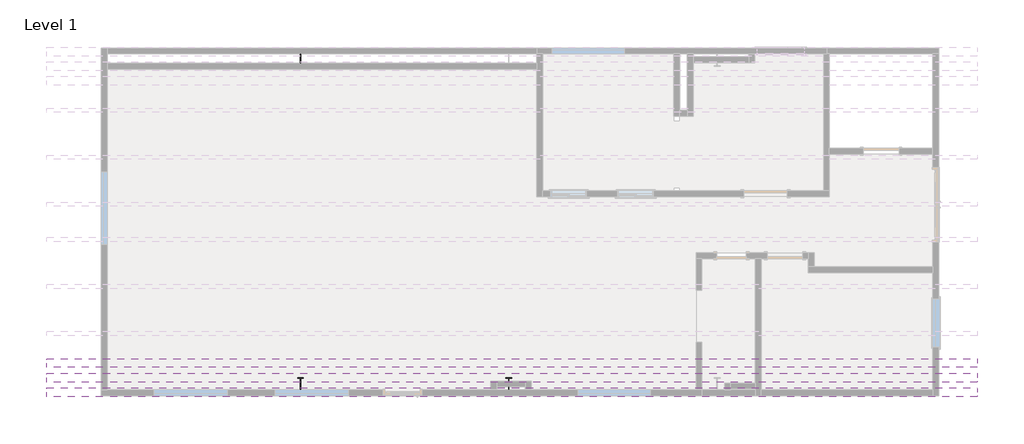
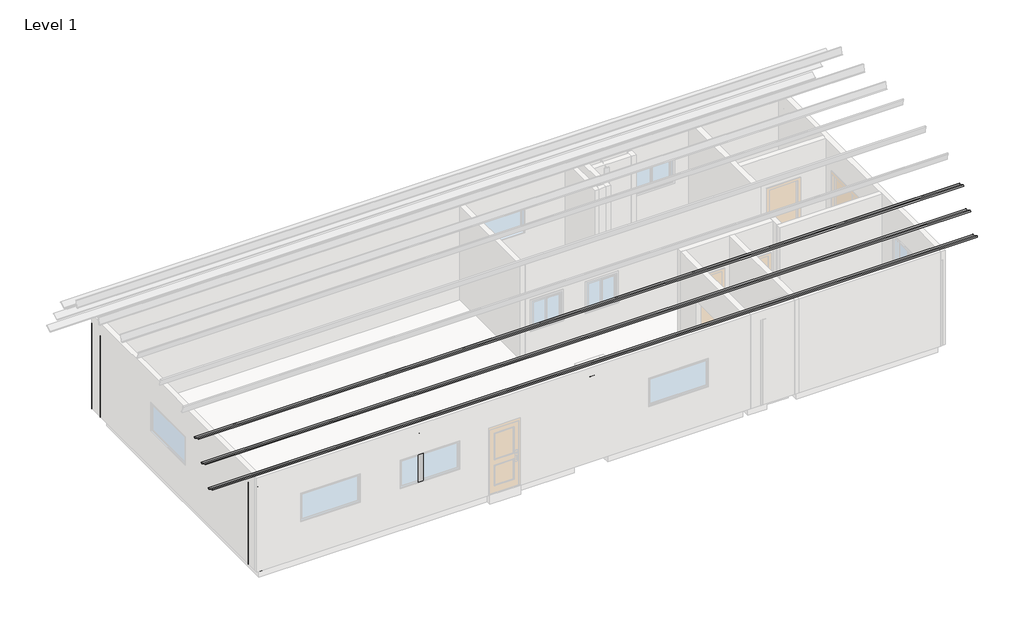
# One storey, part 2 of 3: 5 columns, 3 beams.
"""IFC4 building model written with IfcOpenShell, lengths in millimetres."""

import ifcopenshell
import ifcopenshell.guid

model = None  # the IFC model being written
_history = None  # IfcOwnerHistory: only IFC2X3 demands one
_inside = {}  # id of a spatial element -> (the spatial element, [elements in it])
_under = {}  # id of a project, library or spatial element -> (it, [spatial elements below it])
_declared = {}  # id of a project -> (the project, [libraries it declares])
_typed = {}  # id of a type object -> (the type object, [elements of that type])
_made_of = {}  # id of a material, layer set ... -> (it, [elements and type objects made of it])


def new_model(schema):
    """Start an empty IFC model of exactly this schema.

    Asked for "IFC4X3", IfcOpenShell would pick the latest addendum, in which some entities
    have other attributes; the version numbers below select the first issue.
    IFC2X3 requires an IfcOwnerHistory on every rooted entity: one is made here for all.
    """
    global model, _history
    if schema == "IFC4X3":
        model = ifcopenshell.file(schema_version=(4, 3, 0, 0))
    else:
        model = ifcopenshell.file(schema=schema)
    _inside.clear()
    _under.clear()
    _declared.clear()
    _typed.clear()
    _made_of.clear()
    _history = None
    if model.schema == "IFC2X3":
        org = make("IfcOrganization", Name="unknown")
        user = make(
            "IfcPersonAndOrganization",
            ThePerson=make("IfcPerson", FamilyName="unknown"),
            TheOrganization=org,
        )
        app = make(
            "IfcApplication",
            ApplicationDeveloper=org,
            Version="unknown",
            ApplicationFullName="unknown",
            ApplicationIdentifier="unknown",
        )
        _history = make(
            "IfcOwnerHistory",
            OwningUser=user,
            OwningApplication=app,
            ChangeAction="ADDED",
            CreationDate=0,
        )
    return model


def make(cls, **values):
    """One entity of the class cls with the attributes given. An attribute that is None is left unset."""
    return model.create_entity(
        cls, **{name: value for name, value in values.items() if value is not None}
    )


def rooted(cls, **values):
    """An entity with a GlobalId (a new one), such as an element, a storey or a relation."""
    return make(cls, GlobalId=ifcopenshell.guid.new(), OwnerHistory=_history, **values)


def si_unit(unit_type, name, prefix=None):
    """IfcSIUnit, for example si_unit("LENGTHUNIT", "METRE", prefix="MILLI")."""
    return make("IfcSIUnit", UnitType=unit_type, Prefix=prefix, Name=name)


def assignment(units):
    """IfcUnitAssignment: the units of a project."""
    return None if units is None else make("IfcUnitAssignment", Units=units)


def point(xyz):
    """IfcCartesianPoint."""
    return None if xyz is None else make("IfcCartesianPoint", Coordinates=xyz)


def direction(xyz):
    """IfcDirection."""
    return None if xyz is None else make("IfcDirection", DirectionRatios=xyz)


def frame(location, z_axis=None, x_axis=None):
    """IfcAxis2Placement3D, a coordinate frame: its origin and axes. An axis left out is left unset."""
    return make(
        "IfcAxis2Placement3D",
        Location=point(location),
        Axis=direction(z_axis),
        RefDirection=direction(x_axis),
    )


def origin():
    """The frame at (0, 0, 0) with its axes left unset."""
    return frame((0.0, 0.0, 0.0))


def place(relative_to, where):
    """IfcLocalPlacement: puts the frame where relative to a parent placement (None: the world)."""
    return make(
        "IfcLocalPlacement", PlacementRelTo=relative_to, RelativePlacement=where
    )


def context(
    kind, dimensions, precision=None, world=None, true_north=None, identifier=None
):
    """IfcGeometricRepresentationContext, for example the 3D "Model" context."""
    return make(
        "IfcGeometricRepresentationContext",
        ContextIdentifier=identifier,
        ContextType=kind,
        CoordinateSpaceDimension=dimensions,
        Precision=precision,
        WorldCoordinateSystem=world,
        TrueNorth=true_north,
    )


def project(units=None, contexts=None):
    """IfcProject with its units and contexts."""
    return rooted(
        "IfcProject",
        Name="project",
        RepresentationContexts=contexts,
        UnitsInContext=assignment(units),
    )


def spatial(cls, under=None, at=None, **own):
    """A site, building, storey or space (cls), placed at a placement, below another one or the project."""
    s = rooted(cls, ObjectPlacement=at, **own)
    if under is not None:
        _under.setdefault(under.id(), (under, []))[1].append(s)
    return s


def polyline(points):
    """IfcPolyline through the points."""
    return make("IfcPolyline", Points=[point(p) for p in points])


def circle_curve(where, radius):
    """IfcCircle in the frame where."""
    return make("IfcCircle", Position=where, Radius=radius)


def ellipse_curve(where, semi_axis1, semi_axis2):
    """IfcEllipse in the frame where."""
    return make(
        "IfcEllipse", Position=where, SemiAxis1=semi_axis1, SemiAxis2=semi_axis2
    )


def outline(outer, holes=None, kind="AREA"):
    """IfcArbitraryClosedProfileDef: a profile drawn as a closed curve; with holes, ...WithVoids."""
    if holes is None:
        return make("IfcArbitraryClosedProfileDef", ProfileType=kind, OuterCurve=outer)
    return make(
        "IfcArbitraryProfileDefWithVoids",
        ProfileType=kind,
        OuterCurve=outer,
        InnerCurves=holes,
    )


def extrude(swept, where, along, depth):
    """IfcExtrudedAreaSolid: the profile swept, set in the frame where, extruded along a direction by depth."""
    return make(
        "IfcExtrudedAreaSolid",
        SweptArea=swept,
        Position=where,
        ExtrudedDirection=direction(along),
        Depth=depth,
    )


def shape(context_of_items, identifier, shape_type, items):
    """IfcShapeRepresentation: the items that make up one representation, for example the "Body"."""
    return make(
        "IfcShapeRepresentation",
        ContextOfItems=context_of_items,
        RepresentationIdentifier=identifier,
        RepresentationType=shape_type,
        Items=items,
    )


def source(mapping_origin, context_of_items, identifier, shape_type, items):
    """IfcRepresentationMap: a shape defined once, which mapped items show again and again."""
    return make(
        "IfcRepresentationMap",
        MappingOrigin=mapping_origin,
        MappedRepresentation=shape(context_of_items, identifier, shape_type, items),
    )


def transform(
    local_origin,
    x_axis=None,
    y_axis=None,
    z_axis=None,
    scale=None,
    scale2=None,
    scale3=None,
    uniform=True,
):
    """IfcCartesianTransformationOperator3D, or its non-uniform kind. x_axis, y_axis, z_axis: its Axis1, 2, 3."""
    if uniform:
        return make(
            "IfcCartesianTransformationOperator3D",
            Axis1=direction(x_axis),
            Axis2=direction(y_axis),
            LocalOrigin=point(local_origin),
            Scale=scale,
            Axis3=direction(z_axis),
        )
    return make(
        "IfcCartesianTransformationOperator3DnonUniform",
        Axis1=direction(x_axis),
        Axis2=direction(y_axis),
        LocalOrigin=point(local_origin),
        Scale=scale,
        Axis3=direction(z_axis),
        Scale2=scale2,
        Scale3=scale3,
    )


def mapped(mapping_source, mapping_target):
    """IfcMappedItem: shows the shape of a source again, moved by a transform."""
    return make(
        "IfcMappedItem", MappingSource=mapping_source, MappingTarget=mapping_target
    )


def made_of(thing, what):
    """Note that an element or type object is made of a material, layer set ...; save() writes the relation."""
    if what is not None:
        _made_of.setdefault(what.id(), (what, []))[1].append(thing)
    return thing


def element(
    cls,
    number,
    at=None,
    inside=None,
    cuts=None,
    type_object=None,
    material=None,
    context=None,
    identifier="Body",
    shape_type=None,
    held_by="IfcProductDefinitionShape",
    body=None,
    shapes=None,
    **own,
):
    """One element of the class cls, such as IfcWall. Its Tag is "e" and its number.

    at: its placement. inside: the storey or other place that contains it. cuts: it is an
    opening in that element (IfcRelVoidsElement). A single representation is given by context,
    identifier, shape_type and body (its items); several are given by shapes. held_by: the class
    of the entity that holds the representations. save() writes the other relations.
    """
    e = rooted(cls, Tag="e%d" % number, ObjectPlacement=at, **own)
    if body is not None:
        shapes = [shape(context, identifier, shape_type, body)]
    if shapes is not None:
        e.Representation = make(held_by, Representations=shapes)
    if inside is not None:
        _inside.setdefault(inside.id(), (inside, []))[1].append(e)
    if cuts is not None:
        rooted(
            "IfcRelVoidsElement", RelatingBuildingElement=cuts, RelatedOpeningElement=e
        )
    if type_object is not None:
        _typed.setdefault(type_object.id(), (type_object, []))[1].append(e)
    return made_of(e, material)


def aggregate(whole, parts):
    """IfcRelAggregates: a whole, such as a stair, and the parts it consists of."""
    return rooted("IfcRelAggregates", RelatingObject=whole, RelatedObjects=parts)


def save(model, path):
    """Write the relations noted so far, then the file.

    IfcRelAggregates (storeys below a building ...), IfcRelContainedInSpatialStructure (elements
    in a storey), IfcRelDefinesByType, IfcRelAssociatesMaterial and IfcRelDeclares: one each for
    every whole, place, type object, material and project.
    """
    for whole, parts in _under.values():
        aggregate(whole, parts)
    for where, things in _inside.values():
        rooted(
            "IfcRelContainedInSpatialStructure",
            RelatedElements=things,
            RelatingStructure=where,
        )
    for kind, things in _typed.values():
        rooted("IfcRelDefinesByType", RelatedObjects=things, RelatingType=kind)
    for what, things in _made_of.values():
        rooted("IfcRelAssociatesMaterial", RelatedObjects=things, RelatingMaterial=what)
    for by, libraries in _declared.values():
        rooted("IfcRelDeclares", RelatingContext=by, RelatedDefinitions=libraries)
    model.write(path)


def plane_surface(at):
    """IfcPlane: the flat surface through the origin of the frame at, square to its z axis."""
    return make("IfcPlane", Position=at)


def revolved_surface(curve, axis_point, axis_direction):
    """IfcSurfaceOfRevolution: the curve turned about the line through axis_point along axis_direction."""
    return make(
        "IfcSurfaceOfRevolution",
        SweptCurve=make("IfcArbitraryOpenProfileDef", ProfileType="CURVE", Curve=curve),
        AxisPosition=make("IfcAxis1Placement", Location=point(axis_point), Axis=direction(axis_direction)),
    )


def advanced_brep(points, edges, surfaces, faces):
    """IfcAdvancedBrep: a solid bounded by faces that lie on surfaces and meet in shared edges.

    An edge is (start, end): straight between two places in points (the first is 0);
    or (start, end, curve); or (start, end, curve, False) where it runs against its curve.
    A face is (place in surfaces, loops), or (place, loops, False) where it looks against
    its surface's normal. A loop lists edges by number (the first is 1), with a minus sign
    where the edge is run from its end to its start. The first loop is the outer one.
    """
    corners = [point(p) for p in points]
    vertices = [make("IfcVertexPoint", VertexGeometry=c) for c in corners]
    made = []
    for start, end, *more in edges:
        made.append(
            make(
                "IfcEdgeCurve",
                EdgeStart=vertices[start],
                EdgeEnd=vertices[end],
                EdgeGeometry=more[0] if more else make("IfcPolyline", Points=[corners[start], corners[end]]),
                SameSense=more[1] if len(more) > 1 else True,
            )
        )
    hull = []
    for where, loops, *sense in faces:
        bounds = []
        for j, loop in enumerate(loops):
            ring = [make("IfcOrientedEdge", EdgeElement=made[abs(k) - 1], Orientation=k > 0) for k in loop]
            bounds.append(
                make(
                    "IfcFaceOuterBound" if j == 0 else "IfcFaceBound",
                    Bound=make("IfcEdgeLoop", EdgeList=ring),
                    Orientation=True,
                )
            )
        hull.append(make("IfcAdvancedFace", Bounds=bounds, FaceSurface=surfaces[where], SameSense=sense[0] if sense else True))
    return make("IfcAdvancedBrep", Outer=make("IfcClosedShell", CfsFaces=hull))


def z_shapes_z_3x8_0ff4bf34(model_context):
    return source(origin(), model_context, "Body", "SweptSolid", [
        extrude(outline(polyline([(-57.2805719, 101.596825), (-57.2805719, 111.248825), (-19.1805719, 111.248825), (-19.1805719, -101.603175), (18.9194281, -101.603175), (18.9194281, -107.953175), (-27.1991352, -107.953175), (-27.1991352, 101.596825), (-57.2805719, 101.596825)])), frame((-11963.4, 0.0, 0.0), z_axis=(1.0, 0.0, 0.0), x_axis=(0.0, 1.0, 0.0)), (0.0, 0.0, 1.0), 23926.8),
    ])


model = new_model("IFC4")

# Units and contexts
model_context = context("Model", 3, world=origin())
ifc_project = project(units=[si_unit("LENGTHUNIT", "METRE", prefix="MILLI")], contexts=[model_context])

# Site, building, storey
site = spatial("IfcSite", under=ifc_project)
building = spatial("IfcBuilding", under=site)
storey = spatial("IfcBuildingStorey", under=building, Name="Level 1", Elevation=0.0)

# Beams
placement = place(None, origin())
z_shapes_z_3x8_shape = z_shapes_z_3x8_0ff4bf34(model_context)
element("IfcBeam", 1, ObjectType="Z Shapes : Z 3X8", at=placement, inside=storey, context=model_context, shape_type="MappedRepresentation", body=[
    mapped(z_shapes_z_3x8_shape, transform((18060.1870052, 3496.8149514, 4436.794501), x_axis=(1.0, 0.0, 0.0), y_axis=(0.0, 0.5198738321222879, 0.8542430559708913), z_axis=(0.0, -0.8542430559708913, 0.5198738321222879))),
])
element("IfcBeam", 2, ObjectType="Z Shapes : Z 3X8", at=placement, inside=storey, context=model_context, shape_type="MappedRepresentation", body=[
    mapped(z_shapes_z_3x8_shape, transform((18060.1870052, 3122.2539613, 3821.3256987), x_axis=(1.0, 0.0, 0.0), y_axis=(0.0, 0.5198738321222879, 0.8542430559708913), z_axis=(0.0, -0.8542430559708913, 0.5198738321222879))),
])
element("IfcBeam", 3, ObjectType="Z Shapes : Z 3X8", at=placement, inside=storey, context=model_context, shape_type="MappedRepresentation", body=[
    mapped(z_shapes_z_3x8_shape, transform((18060.1870052, 2747.6929713, 3205.8568965), x_axis=(1.0, 0.0, 0.0), y_axis=(0.0, 0.5198738321222879, 0.8542430559708913), z_axis=(0.0, -0.8542430559708913, 0.5198738321222879))),
])

# Columns
element("IfcColumn", 4, ObjectType="W-Wide Flange-Column : W6X18.5", at=placement, inside=storey, context=model_context, shape_type="AdvancedBrep", body=[
    advanced_brep(
    [(17901.4370052, 2642.8615366, 0.0), (17901.4370052, 2653.1485366, 0.0), (17962.3970052, 2653.1485366, 0.0), (17974.3350052, 2665.0865366, 0.0), (17974.3350052, 3090.5365366, 0.0), (17962.3970052, 3102.4745366, 0.0), (17901.4370052, 3102.4745366, 0.0), (17901.4370052, 3112.7615366, 0.0), (18053.8370052, 3112.7615366, 0.0), (18053.8370052, 3102.4745366, 0.0), (17992.8770052, 3102.4745366, 0.0), (17980.9390052, 3090.5365366, 0.0), (17980.9390052, 2665.0865366, 0.0), (17992.8770052, 2653.1485366, 0.0), (18053.8370052, 2653.1485366, 0.0), (18053.8370052, 2642.8615366, 0.0), (17901.4370052, 2642.8615366, 2825.947988), (17901.4370052, 2653.1485366, 2823.0639572), (17962.3970052, 2653.1485366, 2823.0639572), (17974.3350052, 2665.0865366, 2819.7170571), (17974.3350052, 3090.5365366, 2700.4392375), (17962.3970052, 3102.4745366, 2697.0923375), (17901.4370052, 3102.4745366, 2697.0923375), (17901.4370052, 3112.7615366, 2694.2083066), (18053.8370052, 3112.7615366, 2694.2083066), (18053.8370052, 3102.4745366, 2697.0923375), (17992.8770052, 3102.4745366, 2697.0923375), (17980.9390052, 3090.5365366, 2700.4392375), (17980.9390052, 2665.0865366, 2819.7170571), (17992.8770052, 2653.1485366, 2823.0639572), (18053.8370052, 2653.1485366, 2823.0639572), (18053.8370052, 2642.8615366, 2825.947988)],
    [
        (0, 1),
        (1, 2),
        (2, 3, circle_curve(frame((17962.3970052, 2665.0865366, 0.0), z_axis=(0.0, 0.0, 1.0), x_axis=(-1.0, 0.0, 0.0)), 11.938)),
        (3, 4),
        (4, 5, circle_curve(frame((17962.3970052, 3090.5365366, 0.0), z_axis=(0.0, 0.0, 1.0), x_axis=(-1.0, 0.0, 0.0)), 11.938)),
        (5, 6),
        (6, 7),
        (7, 8),
        (8, 9),
        (9, 10),
        (10, 11, circle_curve(frame((17992.8770052, 3090.5365366, 0.0), z_axis=(0.0, 0.0, 1.0), x_axis=(-1.0, 0.0, 0.0)), 11.938)),
        (11, 12),
        (12, 13, circle_curve(frame((17992.8770052, 2665.0865366, 0.0), z_axis=(0.0, 0.0, 1.0), x_axis=(-1.0, 0.0, 0.0)), 11.938)),
        (13, 14),
        (14, 15),
        (15, 0),
        (0, 16),
        (16, 17),
        (17, 1),
        (17, 18),
        (18, 2),
        (18, 19, ellipse_curve(frame((17962.3970052, 2665.0865366, 2819.7170571), z_axis=(0.0, 0.2699485280248201, 0.962874754169634), x_axis=(0.0, 0.962874754169634, -0.26994852802481967)), 12.3982895, 11.938)),
        (19, 3),
        (19, 20),
        (20, 4),
        (20, 21, ellipse_curve(frame((17962.3970052, 3090.5365366, 2700.4392375), z_axis=(0.0, 0.2699485280248201, 0.962874754169634), x_axis=(0.0, 0.962874754169634, -0.26994852802481967)), 12.3982895, 11.938)),
        (21, 5),
        (21, 22),
        (22, 6),
        (22, 23),
        (23, 7),
        (23, 24),
        (24, 8),
        (24, 25),
        (25, 9),
        (25, 26),
        (26, 10),
        (26, 27, ellipse_curve(frame((17992.8770052, 3090.5365366, 2700.4392375), z_axis=(0.0, 0.2699485280248201, 0.962874754169634), x_axis=(0.0, 0.962874754169634, -0.26994852802481967)), 12.3982895, 11.938)),
        (27, 11),
        (27, 28),
        (28, 12),
        (28, 29, ellipse_curve(frame((17992.8770052, 2665.0865366, 2819.7170571), z_axis=(0.0, 0.2699485280248201, 0.962874754169634), x_axis=(0.0, 0.962874754169634, -0.26994852802481967)), 12.3982895, 11.938)),
        (29, 13),
        (29, 30),
        (30, 14),
        (30, 31),
        (31, 15),
        (31, 16),
    ],
    [
        plane_surface(frame((18053.8370052, 2642.8615366, 0.0), z_axis=(0.0, 0.0, -1.0), x_axis=(-1.0, 0.0, 0.0))),
        plane_surface(frame((17901.4370052, 2653.1485366, 2832.1), z_axis=(-1.0, 0.0, 0.0), x_axis=(0.0, 0.0, -1.0))),
        plane_surface(frame((17962.3970052, 2653.1485366, 2832.1), z_axis=(0.0, 1.0, 0.0), x_axis=(0.0, 0.0, -1.0))),
        revolved_surface(polyline([(17950.459005200002, 2665.0865366, 0.0), (17950.459005200002, 2665.0865366, 2823.0639572)]), (17962.3970052, 2665.0865366, 0.0), (0.0, 0.0, -1.0)),
        plane_surface(frame((17974.3350052, 3090.5365366, 2832.1), z_axis=(-1.0, 0.0, 0.0), x_axis=(0.0, 0.0, -1.0))),
        revolved_surface(polyline([(17950.459005200002, 3090.5365366, 0.0), (17950.459005200002, 3090.5365366, 2703.786137500551)]), (17962.3970052, 3090.5365366, 0.0), (0.0, 0.0, -1.0)),
        plane_surface(frame((17901.4370052, 3102.4745366, 2832.1), z_axis=(0.0, -1.0, 0.0), x_axis=(0.0, 0.0, -1.0))),
        plane_surface(frame((17901.4370052, 3112.7615366, 2832.1), z_axis=(-1.0, 0.0, 0.0), x_axis=(0.0, 0.0, -1.0))),
        plane_surface(frame((18053.8370052, 3112.7615366, 2832.1), z_axis=(0.0, 1.0, 0.0), x_axis=(0.0, 0.0, -1.0))),
        plane_surface(frame((18053.8370052, 3102.4745366, 2832.1), z_axis=(1.0, 0.0, 0.0), x_axis=(0.0, 0.0, -1.0))),
        plane_surface(frame((17992.8770052, 3102.4745366, 2832.1), z_axis=(0.0, -1.0, 0.0), x_axis=(0.0, 0.0, -1.0))),
        revolved_surface(polyline([(17980.9390052, 3090.5365366, 0.0), (17980.9390052, 3090.5365366, 2703.786137500551)]), (17992.8770052, 3090.5365366, 0.0), (0.0, 0.0, -1.0)),
        plane_surface(frame((17980.9390052, 2665.0865366, 2832.1), z_axis=(1.0, 0.0, 0.0), x_axis=(0.0, 0.0, -1.0))),
        revolved_surface(polyline([(17980.9390052, 2665.0865366, 0.0), (17980.9390052, 2665.0865366, 2823.0639572)]), (17992.8770052, 2665.0865366, 0.0), (0.0, 0.0, -1.0)),
        plane_surface(frame((18053.8370052, 2653.1485366, 2832.1), z_axis=(0.0, 1.0, 0.0), x_axis=(0.0, 0.0, -1.0))),
        plane_surface(frame((18053.8370052, 2642.8615366, 2832.1), z_axis=(1.0, 0.0, 0.0), x_axis=(0.0, 0.0, -1.0))),
        plane_surface(frame((17901.4370052, 2642.8615366, 2832.1), z_axis=(0.0, -1.0, 0.0), x_axis=(0.0, 0.0, -1.0))),
        plane_surface(frame((20809.7370052, 2504.5013556, 2864.7382118), z_axis=(0.0, 0.2699485280248201, 0.962874754169634), x_axis=(-1.0, 0.0, 0.0))),
    ],
    [
        (0, [[1, 2, 3, 4, 5, 6, 7, 8, 9, 10, 11, 12, 13, 14, 15, 16]]),
        (1, [[-1, 17, 18, 19]]),
        (2, [[-2, -19, 20, 21]]),
        (3, [[-3, -21, 22, 23]]),
        (4, [[-4, -23, 24, 25]]),
        (5, [[-5, -25, 26, 27]]),
        (6, [[-6, -27, 28, 29]]),
        (7, [[-7, -29, 30, 31]]),
        (8, [[-8, -31, 32, 33]]),
        (9, [[-9, -33, 34, 35]]),
        (10, [[-10, -35, 36, 37]]),
        (11, [[-11, -37, 38, 39]]),
        (12, [[-12, -39, 40, 41]]),
        (13, [[-13, -41, 42, 43]]),
        (14, [[-14, -43, 44, 45]]),
        (15, [[-15, -45, 46, 47]]),
        (16, [[-16, -47, 48, -17]]),
        (17, [[-18, -48, -46, -44, -42, -40, -38, -36, -34, -32, -30, -28, -26, -24, -22, -20]]),
    ],
),
])
element("IfcColumn", 5, ObjectType="W-Wide Flange-Column : W6X18.5", at=placement, inside=storey, context=model_context, shape_type="AdvancedBrep", body=[
    advanced_brep(
    [(12700.7870052, 11583.6615366, 0.0), (12700.7870052, 11573.3745366, 0.0), (12639.8270052, 11573.3745366, 0.0), (12627.8890052, 11561.4365366, 0.0), (12627.8890052, 11135.9865366, 0.0), (12639.8270052, 11124.0485366, 0.0), (12700.7870052, 11124.0485366, 0.0), (12700.7870052, 11113.7615366, 0.0), (12548.3870052, 11113.7615366, 0.0), (12548.3870052, 11124.0485366, 0.0), (12609.3470052, 11124.0485366, 0.0), (12621.2850052, 11135.9865366, 0.0), (12621.2850052, 11561.4365366, 0.0), (12609.3470052, 11573.3745366, 0.0), (12548.3870052, 11573.3745366, 0.0), (12548.3870052, 11583.6615366, 0.0), (12700.7870052, 11583.6615366, 2825.947988), (12700.7870052, 11573.3745366, 2823.0639572), (12639.8270052, 11573.3745366, 2823.0639572), (12627.8890052, 11561.4365366, 2819.7170571), (12627.8890052, 11135.9865366, 2700.4392375), (12639.8270052, 11124.0485366, 2697.0923375), (12700.7870052, 11124.0485366, 2697.0923375), (12700.7870052, 11113.7615366, 2694.2083066), (12548.3870052, 11113.7615366, 2694.2083066), (12548.3870052, 11124.0485366, 2697.0923375), (12609.3470052, 11124.0485366, 2697.0923375), (12621.2850052, 11135.9865366, 2700.4392375), (12621.2850052, 11561.4365366, 2819.7170571), (12609.3470052, 11573.3745366, 2823.0639572), (12548.3870052, 11573.3745366, 2823.0639572), (12548.3870052, 11583.6615366, 2825.947988)],
    [
        (0, 1),
        (1, 2),
        (2, 3, circle_curve(frame((12639.8270052, 11561.4365366, 0.0), z_axis=(0.0, 0.0, 1.0), x_axis=(1.0, 0.0, 0.0)), 11.938)),
        (3, 4),
        (4, 5, circle_curve(frame((12639.8270052, 11135.9865366, 0.0), z_axis=(0.0, 0.0, 1.0), x_axis=(1.0, 0.0, 0.0)), 11.938)),
        (5, 6),
        (6, 7),
        (7, 8),
        (8, 9),
        (9, 10),
        (10, 11, circle_curve(frame((12609.3470052, 11135.9865366, 0.0), z_axis=(0.0, 0.0, 1.0), x_axis=(1.0, 0.0, 0.0)), 11.938)),
        (11, 12),
        (12, 13, circle_curve(frame((12609.3470052, 11561.4365366, 0.0), z_axis=(0.0, 0.0, 1.0), x_axis=(1.0, 0.0, 0.0)), 11.938)),
        (13, 14),
        (14, 15),
        (15, 0),
        (0, 16),
        (16, 17),
        (17, 1),
        (17, 18),
        (18, 2),
        (18, 19, ellipse_curve(frame((12639.8270052, 11561.4365366, 2819.7170571), z_axis=(0.0, -0.26994852802481994, 0.962874754169634), x_axis=(0.0, -0.9628747541696339, -0.26994852802481983)), 12.3982895, 11.938)),
        (19, 3),
        (19, 20),
        (20, 4),
        (20, 21, ellipse_curve(frame((12639.8270052, 11135.9865366, 2700.4392375), z_axis=(0.0, -0.26994852802481994, 0.962874754169634), x_axis=(0.0, -0.9628747541696339, -0.26994852802481983)), 12.3982895, 11.938)),
        (21, 5),
        (21, 22),
        (22, 6),
        (22, 23),
        (23, 7),
        (23, 24),
        (24, 8),
        (24, 25),
        (25, 9),
        (25, 26),
        (26, 10),
        (26, 27, ellipse_curve(frame((12609.3470052, 11135.9865366, 2700.4392375), z_axis=(0.0, -0.26994852802481994, 0.962874754169634), x_axis=(0.0, -0.9628747541696339, -0.26994852802481983)), 12.3982895, 11.938)),
        (27, 11),
        (27, 28),
        (28, 12),
        (28, 29, ellipse_curve(frame((12609.3470052, 11561.4365366, 2819.7170571), z_axis=(0.0, -0.26994852802481994, 0.962874754169634), x_axis=(0.0, -0.9628747541696339, -0.26994852802481983)), 12.3982895, 11.938)),
        (29, 13),
        (29, 30),
        (30, 14),
        (30, 31),
        (31, 15),
        (31, 16),
    ],
    [
        plane_surface(frame((12548.3870052, 11583.6615366, 0.0), z_axis=(0.0, 0.0, -1.0), x_axis=(1.0, 0.0, 0.0))),
        plane_surface(frame((12700.7870052, 11573.3745366, 2832.1), z_axis=(1.0, 0.0, 0.0), x_axis=(0.0, 0.0, -1.0))),
        plane_surface(frame((12639.8270052, 11573.3745366, 2832.1), z_axis=(0.0, -1.0, 0.0), x_axis=(0.0, 0.0, -1.0))),
        revolved_surface(polyline([(12651.7650052, 11561.4365366, 0.0), (12651.7650052, 11561.4365366, 2823.0639572)]), (12639.8270052, 11561.4365366, 0.0), (0.0, 0.0, -1.0)),
        plane_surface(frame((12627.8890052, 11135.9865366, 2832.1), z_axis=(1.0, 0.0, 0.0), x_axis=(0.0, 0.0, -1.0))),
        revolved_surface(polyline([(12651.7650052, 11135.9865366, 0.0), (12651.7650052, 11135.9865366, 2703.786137500551)]), (12639.8270052, 11135.9865366, 0.0), (0.0, 0.0, -1.0)),
        plane_surface(frame((12700.7870052, 11124.0485366, 2832.1), z_axis=(0.0, 1.0, 0.0), x_axis=(0.0, 0.0, -1.0))),
        plane_surface(frame((12700.7870052, 11113.7615366, 2832.1), z_axis=(1.0, 0.0, 0.0), x_axis=(0.0, 0.0, -1.0))),
        plane_surface(frame((12548.3870052, 11113.7615366, 2832.1), z_axis=(0.0, -1.0, 0.0), x_axis=(0.0, 0.0, -1.0))),
        plane_surface(frame((12548.3870052, 11124.0485366, 2832.1), z_axis=(-1.0, 0.0, 0.0), x_axis=(0.0, 0.0, -1.0))),
        plane_surface(frame((12609.3470052, 11124.0485366, 2832.1), z_axis=(0.0, 1.0, 0.0), x_axis=(0.0, 0.0, -1.0))),
        revolved_surface(polyline([(12621.2850052, 11135.9865366, 0.0), (12621.2850052, 11135.9865366, 2703.786137500551)]), (12609.3470052, 11135.9865366, 0.0), (0.0, 0.0, -1.0)),
        plane_surface(frame((12621.2850052, 11561.4365366, 2832.1), z_axis=(-1.0, 0.0, 0.0), x_axis=(0.0, 0.0, -1.0))),
        revolved_surface(polyline([(12621.2850052, 11561.4365366, 0.0), (12621.2850052, 11561.4365366, 2823.0639572)]), (12609.3470052, 11561.4365366, 0.0), (0.0, 0.0, -1.0)),
        plane_surface(frame((12548.3870052, 11573.3745366, 2832.1), z_axis=(0.0, -1.0, 0.0), x_axis=(0.0, 0.0, -1.0))),
        plane_surface(frame((12548.3870052, 11583.6615366, 2832.1), z_axis=(-1.0, 0.0, 0.0), x_axis=(0.0, 0.0, -1.0))),
        plane_surface(frame((12700.7870052, 11583.6615366, 2832.1), z_axis=(0.0, 1.0, 0.0), x_axis=(0.0, 0.0, -1.0))),
        plane_surface(frame((9792.4870052, 11722.0217176, 2864.7382118), z_axis=(0.0, -0.26994852802481994, 0.962874754169634), x_axis=(1.0, 0.0, 0.0))),
    ],
    [
        (0, [[1, 2, 3, 4, 5, 6, 7, 8, 9, 10, 11, 12, 13, 14, 15, 16]]),
        (1, [[-1, 17, 18, 19]]),
        (2, [[-2, -19, 20, 21]]),
        (3, [[-3, -21, 22, 23]]),
        (4, [[-4, -23, 24, 25]]),
        (5, [[-5, -25, 26, 27]]),
        (6, [[-6, -27, 28, 29]]),
        (7, [[-7, -29, 30, 31]]),
        (8, [[-8, -31, 32, 33]]),
        (9, [[-9, -33, 34, 35]]),
        (10, [[-10, -35, 36, 37]]),
        (11, [[-11, -37, 38, 39]]),
        (12, [[-12, -39, 40, 41]]),
        (13, [[-13, -41, 42, 43]]),
        (14, [[-14, -43, 44, 45]]),
        (15, [[-15, -45, 46, 47]]),
        (16, [[-16, -47, 48, -17]]),
        (17, [[-18, -48, -46, -44, -42, -40, -38, -36, -34, -32, -30, -28, -26, -24, -22, -20]]),
    ],
),
])
element("IfcColumn", 6, ObjectType="W-Wide Flange-Column : W6X18.5", at=placement, inside=storey, context=model_context, shape_type="AdvancedBrep", body=[
    advanced_brep(
    [(12548.3870052, 2642.8615366, 0.0), (12548.3870052, 2653.1485366, 0.0), (12609.3470052, 2653.1485366, 0.0), (12621.2850052, 2665.0865366, 0.0), (12621.2850052, 3090.5365366, 0.0), (12609.3470052, 3102.4745366, 0.0), (12548.3870052, 3102.4745366, 0.0), (12548.3870052, 3112.7615366, 0.0), (12700.7870052, 3112.7615366, 0.0), (12700.7870052, 3102.4745366, 0.0), (12639.8270052, 3102.4745366, 0.0), (12627.8890052, 3090.5365366, 0.0), (12627.8890052, 2665.0865366, 0.0), (12639.8270052, 2653.1485366, 0.0), (12700.7870052, 2653.1485366, 0.0), (12700.7870052, 2642.8615366, 0.0), (12548.3870052, 2642.8615366, 2825.947988), (12548.3870052, 2653.1485366, 2823.0639572), (12609.3470052, 2653.1485366, 2823.0639572), (12621.2850052, 2665.0865366, 2819.7170571), (12621.2850052, 3090.5365366, 2700.4392375), (12609.3470052, 3102.4745366, 2697.0923375), (12548.3870052, 3102.4745366, 2697.0923375), (12548.3870052, 3112.7615366, 2694.2083066), (12700.7870052, 3112.7615366, 2694.2083066), (12700.7870052, 3102.4745366, 2697.0923375), (12639.8270052, 3102.4745366, 2697.0923375), (12627.8890052, 3090.5365366, 2700.4392375), (12627.8890052, 2665.0865366, 2819.7170571), (12639.8270052, 2653.1485366, 2823.0639572), (12700.7870052, 2653.1485366, 2823.0639572), (12700.7870052, 2642.8615366, 2825.947988)],
    [
        (0, 1),
        (1, 2),
        (2, 3, circle_curve(frame((12609.3470052, 2665.0865366, 0.0), z_axis=(0.0, 0.0, 1.0), x_axis=(-1.0, 0.0, 0.0)), 11.938)),
        (3, 4),
        (4, 5, circle_curve(frame((12609.3470052, 3090.5365366, 0.0), z_axis=(0.0, 0.0, 1.0), x_axis=(-1.0, 0.0, 0.0)), 11.938)),
        (5, 6),
        (6, 7),
        (7, 8),
        (8, 9),
        (9, 10),
        (10, 11, circle_curve(frame((12639.8270052, 3090.5365366, 0.0), z_axis=(0.0, 0.0, 1.0), x_axis=(-1.0, 0.0, 0.0)), 11.938)),
        (11, 12),
        (12, 13, circle_curve(frame((12639.8270052, 2665.0865366, 0.0), z_axis=(0.0, 0.0, 1.0), x_axis=(-1.0, 0.0, 0.0)), 11.938)),
        (13, 14),
        (14, 15),
        (15, 0),
        (0, 16),
        (16, 17),
        (17, 1),
        (17, 18),
        (18, 2),
        (18, 19, ellipse_curve(frame((12609.3470052, 2665.0865366, 2819.7170571), z_axis=(0.0, 0.2699485280248201, 0.962874754169634), x_axis=(0.0, 0.962874754169634, -0.26994852802481967)), 12.3982895, 11.938)),
        (19, 3),
        (19, 20),
        (20, 4),
        (20, 21, ellipse_curve(frame((12609.3470052, 3090.5365366, 2700.4392375), z_axis=(0.0, 0.2699485280248201, 0.962874754169634), x_axis=(0.0, 0.962874754169634, -0.26994852802481967)), 12.3982895, 11.938)),
        (21, 5),
        (21, 22),
        (22, 6),
        (22, 23),
        (23, 7),
        (23, 24),
        (24, 8),
        (24, 25),
        (25, 9),
        (25, 26),
        (26, 10),
        (26, 27, ellipse_curve(frame((12639.8270052, 3090.5365366, 2700.4392375), z_axis=(0.0, 0.2699485280248201, 0.962874754169634), x_axis=(0.0, 0.962874754169634, -0.26994852802481967)), 12.3982895, 11.938)),
        (27, 11),
        (27, 28),
        (28, 12),
        (28, 29, ellipse_curve(frame((12639.8270052, 2665.0865366, 2819.7170571), z_axis=(0.0, 0.2699485280248201, 0.962874754169634), x_axis=(0.0, 0.962874754169634, -0.26994852802481967)), 12.3982895, 11.938)),
        (29, 13),
        (29, 30),
        (30, 14),
        (30, 31),
        (31, 15),
        (31, 16),
    ],
    [
        plane_surface(frame((12700.7870052, 2642.8615366, 0.0), z_axis=(0.0, 0.0, -1.0), x_axis=(-1.0, 0.0, 0.0))),
        plane_surface(frame((12548.3870052, 2653.1485366, 2832.1), z_axis=(-1.0, 0.0, 0.0), x_axis=(0.0, 0.0, -1.0))),
        plane_surface(frame((12609.3470052, 2653.1485366, 2832.1), z_axis=(0.0, 1.0, 0.0), x_axis=(0.0, 0.0, -1.0))),
        revolved_surface(polyline([(12597.4090052, 2665.0865366, 0.0), (12597.4090052, 2665.0865366, 2823.0639572)]), (12609.3470052, 2665.0865366, 0.0), (0.0, 0.0, -1.0)),
        plane_surface(frame((12621.2850052, 3090.5365366, 2832.1), z_axis=(-1.0, 0.0, 0.0), x_axis=(0.0, 0.0, -1.0))),
        revolved_surface(polyline([(12597.4090052, 3090.5365366, 0.0), (12597.4090052, 3090.5365366, 2703.786137500551)]), (12609.3470052, 3090.5365366, 0.0), (0.0, 0.0, -1.0)),
        plane_surface(frame((12548.3870052, 3102.4745366, 2832.1), z_axis=(0.0, -1.0, 0.0), x_axis=(0.0, 0.0, -1.0))),
        plane_surface(frame((12548.3870052, 3112.7615366, 2832.1), z_axis=(-1.0, 0.0, 0.0), x_axis=(0.0, 0.0, -1.0))),
        plane_surface(frame((12700.7870052, 3112.7615366, 2832.1), z_axis=(0.0, 1.0, 0.0), x_axis=(0.0, 0.0, -1.0))),
        plane_surface(frame((12700.7870052, 3102.4745366, 2832.1), z_axis=(1.0, 0.0, 0.0), x_axis=(0.0, 0.0, -1.0))),
        plane_surface(frame((12639.8270052, 3102.4745366, 2832.1), z_axis=(0.0, -1.0, 0.0), x_axis=(0.0, 0.0, -1.0))),
        revolved_surface(polyline([(12627.8890052, 3090.5365366, 0.0), (12627.8890052, 3090.5365366, 2703.786137500551)]), (12639.8270052, 3090.5365366, 0.0), (0.0, 0.0, -1.0)),
        plane_surface(frame((12627.8890052, 2665.0865366, 2832.1), z_axis=(1.0, 0.0, 0.0), x_axis=(0.0, 0.0, -1.0))),
        revolved_surface(polyline([(12627.8890052, 2665.0865366, 0.0), (12627.8890052, 2665.0865366, 2823.0639572)]), (12639.8270052, 2665.0865366, 0.0), (0.0, 0.0, -1.0)),
        plane_surface(frame((12700.7870052, 2653.1485366, 2832.1), z_axis=(0.0, 1.0, 0.0), x_axis=(0.0, 0.0, -1.0))),
        plane_surface(frame((12700.7870052, 2642.8615366, 2832.1), z_axis=(1.0, 0.0, 0.0), x_axis=(0.0, 0.0, -1.0))),
        plane_surface(frame((12548.3870052, 2642.8615366, 2832.1), z_axis=(0.0, -1.0, 0.0), x_axis=(0.0, 0.0, -1.0))),
        plane_surface(frame((15456.6870052, 2504.5013556, 2864.7382118), z_axis=(0.0, 0.2699485280248201, 0.962874754169634), x_axis=(-1.0, 0.0, 0.0))),
    ],
    [
        (0, [[1, 2, 3, 4, 5, 6, 7, 8, 9, 10, 11, 12, 13, 14, 15, 16]]),
        (1, [[-1, 17, 18, 19]]),
        (2, [[-2, -19, 20, 21]]),
        (3, [[-3, -21, 22, 23]]),
        (4, [[-4, -23, 24, 25]]),
        (5, [[-5, -25, 26, 27]]),
        (6, [[-6, -27, 28, 29]]),
        (7, [[-7, -29, 30, 31]]),
        (8, [[-8, -31, 32, 33]]),
        (9, [[-9, -33, 34, 35]]),
        (10, [[-10, -35, 36, 37]]),
        (11, [[-11, -37, 38, 39]]),
        (12, [[-12, -39, 40, 41]]),
        (13, [[-13, -41, 42, 43]]),
        (14, [[-14, -43, 44, 45]]),
        (15, [[-15, -45, 46, 47]]),
        (16, [[-16, -47, 48, -17]]),
        (17, [[-18, -48, -46, -44, -42, -40, -38, -36, -34, -32, -30, -28, -26, -24, -22, -20]]),
    ],
),
])
element("IfcColumn", 7, ObjectType="W-Wide Flange-Column : W6X18.5", at=placement, inside=storey, context=model_context, shape_type="AdvancedBrep", body=[
    advanced_brep(
    [(7652.5405771, 11583.6615366, 0.0), (7652.5405771, 11573.3745366, 0.0), (7591.5805771, 11573.3745366, 0.0), (7579.6425771, 11561.4365366, 0.0), (7579.6425771, 11135.9865366, 0.0), (7591.5805771, 11124.0485366, 0.0), (7652.5405771, 11124.0485366, 0.0), (7652.5405771, 11113.7615366, 0.0), (7500.1405771, 11113.7615366, 0.0), (7500.1405771, 11124.0485366, 0.0), (7561.1005771, 11124.0485366, 0.0), (7573.0385771, 11135.9865366, 0.0), (7573.0385771, 11561.4365366, 0.0), (7561.1005771, 11573.3745366, 0.0), (7500.1405771, 11573.3745366, 0.0), (7500.1405771, 11583.6615366, 0.0), (7652.5405771, 11583.6615366, 2825.947988), (7652.5405771, 11573.3745366, 2823.0639572), (7591.5805771, 11573.3745366, 2823.0639572), (7579.6425771, 11561.4365366, 2819.7170571), (7579.6425771, 11135.9865366, 2700.4392375), (7591.5805771, 11124.0485366, 2697.0923375), (7652.5405771, 11124.0485366, 2697.0923375), (7652.5405771, 11113.7615366, 2694.2083066), (7500.1405771, 11113.7615366, 2694.2083066), (7500.1405771, 11124.0485366, 2697.0923375), (7561.1005771, 11124.0485366, 2697.0923375), (7573.0385771, 11135.9865366, 2700.4392375), (7573.0385771, 11561.4365366, 2819.7170571), (7561.1005771, 11573.3745366, 2823.0639572), (7500.1405771, 11573.3745366, 2823.0639572), (7500.1405771, 11583.6615366, 2825.947988)],
    [
        (0, 1),
        (1, 2),
        (2, 3, circle_curve(frame((7591.5805771, 11561.4365366, 0.0), z_axis=(0.0, 0.0, 1.0), x_axis=(1.0, 0.0, 0.0)), 11.938)),
        (3, 4),
        (4, 5, circle_curve(frame((7591.5805771, 11135.9865366, 0.0), z_axis=(0.0, 0.0, 1.0), x_axis=(1.0, 0.0, 0.0)), 11.938)),
        (5, 6),
        (6, 7),
        (7, 8),
        (8, 9),
        (9, 10),
        (10, 11, circle_curve(frame((7561.1005771, 11135.9865366, 0.0), z_axis=(0.0, 0.0, 1.0), x_axis=(1.0, 0.0, 0.0)), 11.938)),
        (11, 12),
        (12, 13, circle_curve(frame((7561.1005771, 11561.4365366, 0.0), z_axis=(0.0, 0.0, 1.0), x_axis=(1.0, 0.0, 0.0)), 11.938)),
        (13, 14),
        (14, 15),
        (15, 0),
        (0, 16),
        (16, 17),
        (17, 1),
        (17, 18),
        (18, 2),
        (18, 19, ellipse_curve(frame((7591.5805771, 11561.4365366, 2819.7170571), z_axis=(0.0, -0.26994852802481994, 0.962874754169634), x_axis=(0.0, -0.9628747541696339, -0.26994852802481983)), 12.3982895, 11.938)),
        (19, 3),
        (19, 20),
        (20, 4),
        (20, 21, ellipse_curve(frame((7591.5805771, 11135.9865366, 2700.4392375), z_axis=(0.0, -0.26994852802481994, 0.962874754169634), x_axis=(0.0, -0.9628747541696339, -0.26994852802481983)), 12.3982895, 11.938)),
        (21, 5),
        (21, 22),
        (22, 6),
        (22, 23),
        (23, 7),
        (23, 24),
        (24, 8),
        (24, 25),
        (25, 9),
        (25, 26),
        (26, 10),
        (26, 27, ellipse_curve(frame((7561.1005771, 11135.9865366, 2700.4392375), z_axis=(0.0, -0.26994852802481994, 0.962874754169634), x_axis=(0.0, -0.9628747541696339, -0.26994852802481983)), 12.3982895, 11.938)),
        (27, 11),
        (27, 28),
        (28, 12),
        (28, 29, ellipse_curve(frame((7561.1005771, 11561.4365366, 2819.7170571), z_axis=(0.0, -0.26994852802481994, 0.962874754169634), x_axis=(0.0, -0.9628747541696339, -0.26994852802481983)), 12.3982895, 11.938)),
        (29, 13),
        (29, 30),
        (30, 14),
        (30, 31),
        (31, 15),
        (31, 16),
    ],
    [
        plane_surface(frame((7500.1405771, 11583.6615366, 0.0), z_axis=(0.0, 0.0, -1.0), x_axis=(1.0, 0.0, 0.0))),
        plane_surface(frame((7652.5405771, 11573.3745366, 2832.1), z_axis=(1.0, 0.0, 0.0), x_axis=(0.0, 0.0, -1.0))),
        plane_surface(frame((7591.5805771, 11573.3745366, 2832.1), z_axis=(0.0, -1.0, 0.0), x_axis=(0.0, 0.0, -1.0))),
        revolved_surface(polyline([(7603.5185771, 11561.4365366, 0.0), (7603.5185771, 11561.4365366, 2823.0639572)]), (7591.5805771, 11561.4365366, 0.0), (0.0, 0.0, -1.0)),
        plane_surface(frame((7579.6425771, 11135.9865366, 2832.1), z_axis=(1.0, 0.0, 0.0), x_axis=(0.0, 0.0, -1.0))),
        revolved_surface(polyline([(7603.5185771, 11135.9865366, 0.0), (7603.5185771, 11135.9865366, 2703.786137500551)]), (7591.5805771, 11135.9865366, 0.0), (0.0, 0.0, -1.0)),
        plane_surface(frame((7652.5405771, 11124.0485366, 2832.1), z_axis=(0.0, 1.0, 0.0), x_axis=(0.0, 0.0, -1.0))),
        plane_surface(frame((7652.5405771, 11113.7615366, 2832.1), z_axis=(1.0, 0.0, 0.0), x_axis=(0.0, 0.0, -1.0))),
        plane_surface(frame((7500.1405771, 11113.7615366, 2832.1), z_axis=(0.0, -1.0, 0.0), x_axis=(0.0, 0.0, -1.0))),
        plane_surface(frame((7500.1405771, 11124.0485366, 2832.1), z_axis=(-1.0, 0.0, 0.0), x_axis=(0.0, 0.0, -1.0))),
        plane_surface(frame((7561.1005771, 11124.0485366, 2832.1), z_axis=(0.0, 1.0, 0.0), x_axis=(0.0, 0.0, -1.0))),
        revolved_surface(polyline([(7573.0385771, 11135.9865366, 0.0), (7573.0385771, 11135.9865366, 2703.786137500551)]), (7561.1005771, 11135.9865366, 0.0), (0.0, 0.0, -1.0)),
        plane_surface(frame((7573.0385771, 11561.4365366, 2832.1), z_axis=(-1.0, 0.0, 0.0), x_axis=(0.0, 0.0, -1.0))),
        revolved_surface(polyline([(7573.0385771, 11561.4365366, 0.0), (7573.0385771, 11561.4365366, 2823.0639572)]), (7561.1005771, 11561.4365366, 0.0), (0.0, 0.0, -1.0)),
        plane_surface(frame((7500.1405771, 11573.3745366, 2832.1), z_axis=(0.0, -1.0, 0.0), x_axis=(0.0, 0.0, -1.0))),
        plane_surface(frame((7500.1405771, 11583.6615366, 2832.1), z_axis=(-1.0, 0.0, 0.0), x_axis=(0.0, 0.0, -1.0))),
        plane_surface(frame((7652.5405771, 11583.6615366, 2832.1), z_axis=(0.0, 1.0, 0.0), x_axis=(0.0, 0.0, -1.0))),
        plane_surface(frame((4744.2405771, 11722.0217176, 2864.7382118), z_axis=(0.0, -0.26994852802481994, 0.962874754169634), x_axis=(1.0, 0.0, 0.0))),
    ],
    [
        (0, [[1, 2, 3, 4, 5, 6, 7, 8, 9, 10, 11, 12, 13, 14, 15, 16]]),
        (1, [[-1, 17, 18, 19]]),
        (2, [[-2, -19, 20, 21]]),
        (3, [[-3, -21, 22, 23]]),
        (4, [[-4, -23, 24, 25]]),
        (5, [[-5, -25, 26, 27]]),
        (6, [[-6, -27, 28, 29]]),
        (7, [[-7, -29, 30, 31]]),
        (8, [[-8, -31, 32, 33]]),
        (9, [[-9, -33, 34, 35]]),
        (10, [[-10, -35, 36, 37]]),
        (11, [[-11, -37, 38, 39]]),
        (12, [[-12, -39, 40, 41]]),
        (13, [[-13, -41, 42, 43]]),
        (14, [[-14, -43, 44, 45]]),
        (15, [[-15, -45, 46, 47]]),
        (16, [[-16, -47, 48, -17]]),
        (17, [[-18, -48, -46, -44, -42, -40, -38, -36, -34, -32, -30, -28, -26, -24, -22, -20]]),
    ],
),
])
element("IfcColumn", 8, ObjectType="W-Wide Flange-Column : W6X18.5", at=placement, inside=storey, context=model_context, shape_type="AdvancedBrep", body=[
    advanced_brep(
    [(7500.1405771, 2642.8615366, 0.0), (7500.1405771, 2653.1485366, 0.0), (7561.1005771, 2653.1485366, 0.0), (7573.0385771, 2665.0865366, 0.0), (7573.0385771, 3090.5365366, 0.0), (7561.1005771, 3102.4745366, 0.0), (7500.1405771, 3102.4745366, 0.0), (7500.1405771, 3112.7615366, 0.0), (7652.5405771, 3112.7615366, 0.0), (7652.5405771, 3102.4745366, 0.0), (7591.5805771, 3102.4745366, 0.0), (7579.6425771, 3090.5365366, 0.0), (7579.6425771, 2665.0865366, 0.0), (7591.5805771, 2653.1485366, 0.0), (7652.5405771, 2653.1485366, 0.0), (7652.5405771, 2642.8615366, 0.0), (7500.1405771, 2642.8615366, 2825.947988), (7500.1405771, 2653.1485366, 2823.0639572), (7561.1005771, 2653.1485366, 2823.0639572), (7573.0385771, 2665.0865366, 2819.7170571), (7573.0385771, 3090.5365366, 2700.4392375), (7561.1005771, 3102.4745366, 2697.0923375), (7500.1405771, 3102.4745366, 2697.0923375), (7500.1405771, 3112.7615366, 2694.2083066), (7652.5405771, 3112.7615366, 2694.2083066), (7652.5405771, 3102.4745366, 2697.0923375), (7591.5805771, 3102.4745366, 2697.0923375), (7579.6425771, 3090.5365366, 2700.4392375), (7579.6425771, 2665.0865366, 2819.7170571), (7591.5805771, 2653.1485366, 2823.0639572), (7652.5405771, 2653.1485366, 2823.0639572), (7652.5405771, 2642.8615366, 2825.947988)],
    [
        (0, 1),
        (1, 2),
        (2, 3, circle_curve(frame((7561.1005771, 2665.0865366, 0.0), z_axis=(0.0, 0.0, 1.0), x_axis=(-1.0, 0.0, 0.0)), 11.938)),
        (3, 4),
        (4, 5, circle_curve(frame((7561.1005771, 3090.5365366, 0.0), z_axis=(0.0, 0.0, 1.0), x_axis=(-1.0, 0.0, 0.0)), 11.938)),
        (5, 6),
        (6, 7),
        (7, 8),
        (8, 9),
        (9, 10),
        (10, 11, circle_curve(frame((7591.5805771, 3090.5365366, 0.0), z_axis=(0.0, 0.0, 1.0), x_axis=(-1.0, 0.0, 0.0)), 11.938)),
        (11, 12),
        (12, 13, circle_curve(frame((7591.5805771, 2665.0865366, 0.0), z_axis=(0.0, 0.0, 1.0), x_axis=(-1.0, 0.0, 0.0)), 11.938)),
        (13, 14),
        (14, 15),
        (15, 0),
        (0, 16),
        (16, 17),
        (17, 1),
        (17, 18),
        (18, 2),
        (18, 19, ellipse_curve(frame((7561.1005771, 2665.0865366, 2819.7170571), z_axis=(0.0, 0.2699485280248201, 0.962874754169634), x_axis=(0.0, 0.962874754169634, -0.26994852802481967)), 12.3982895, 11.938)),
        (19, 3),
        (19, 20),
        (20, 4),
        (20, 21, ellipse_curve(frame((7561.1005771, 3090.5365366, 2700.4392375), z_axis=(0.0, 0.2699485280248201, 0.962874754169634), x_axis=(0.0, 0.962874754169634, -0.26994852802481967)), 12.3982895, 11.938)),
        (21, 5),
        (21, 22),
        (22, 6),
        (22, 23),
        (23, 7),
        (23, 24),
        (24, 8),
        (24, 25),
        (25, 9),
        (25, 26),
        (26, 10),
        (26, 27, ellipse_curve(frame((7591.5805771, 3090.5365366, 2700.4392375), z_axis=(0.0, 0.2699485280248201, 0.962874754169634), x_axis=(0.0, 0.962874754169634, -0.26994852802481967)), 12.3982895, 11.938)),
        (27, 11),
        (27, 28),
        (28, 12),
        (28, 29, ellipse_curve(frame((7591.5805771, 2665.0865366, 2819.7170571), z_axis=(0.0, 0.2699485280248201, 0.962874754169634), x_axis=(0.0, 0.962874754169634, -0.26994852802481967)), 12.3982895, 11.938)),
        (29, 13),
        (29, 30),
        (30, 14),
        (30, 31),
        (31, 15),
        (31, 16),
    ],
    [
        plane_surface(frame((7652.5405771, 2642.8615366, 0.0), z_axis=(0.0, 0.0, -1.0), x_axis=(-1.0, 0.0, 0.0))),
        plane_surface(frame((7500.1405771, 2653.1485366, 2832.1), z_axis=(-1.0, 0.0, 0.0), x_axis=(0.0, 0.0, -1.0))),
        plane_surface(frame((7561.1005771, 2653.1485366, 2832.1), z_axis=(0.0, 1.0, 0.0), x_axis=(0.0, 0.0, -1.0))),
        revolved_surface(polyline([(7549.1625771, 2665.0865366, 0.0), (7549.1625771, 2665.0865366, 2823.0639572)]), (7561.1005771, 2665.0865366, 0.0), (0.0, 0.0, -1.0)),
        plane_surface(frame((7573.0385771, 3090.5365366, 2832.1), z_axis=(-1.0, 0.0, 0.0), x_axis=(0.0, 0.0, -1.0))),
        revolved_surface(polyline([(7549.1625771, 3090.5365366, 0.0), (7549.1625771, 3090.5365366, 2703.786137500551)]), (7561.1005771, 3090.5365366, 0.0), (0.0, 0.0, -1.0)),
        plane_surface(frame((7500.1405771, 3102.4745366, 2832.1), z_axis=(0.0, -1.0, 0.0), x_axis=(0.0, 0.0, -1.0))),
        plane_surface(frame((7500.1405771, 3112.7615366, 2832.1), z_axis=(-1.0, 0.0, 0.0), x_axis=(0.0, 0.0, -1.0))),
        plane_surface(frame((7652.5405771, 3112.7615366, 2832.1), z_axis=(0.0, 1.0, 0.0), x_axis=(0.0, 0.0, -1.0))),
        plane_surface(frame((7652.5405771, 3102.4745366, 2832.1), z_axis=(1.0, 0.0, 0.0), x_axis=(0.0, 0.0, -1.0))),
        plane_surface(frame((7591.5805771, 3102.4745366, 2832.1), z_axis=(0.0, -1.0, 0.0), x_axis=(0.0, 0.0, -1.0))),
        revolved_surface(polyline([(7579.6425770999995, 3090.5365366, 0.0), (7579.6425770999995, 3090.5365366, 2703.786137500551)]), (7591.5805771, 3090.5365366, 0.0), (0.0, 0.0, -1.0)),
        plane_surface(frame((7579.6425771, 2665.0865366, 2832.1), z_axis=(1.0, 0.0, 0.0), x_axis=(0.0, 0.0, -1.0))),
        revolved_surface(polyline([(7579.6425770999995, 2665.0865366, 0.0), (7579.6425770999995, 2665.0865366, 2823.0639572)]), (7591.5805771, 2665.0865366, 0.0), (0.0, 0.0, -1.0)),
        plane_surface(frame((7652.5405771, 2653.1485366, 2832.1), z_axis=(0.0, 1.0, 0.0), x_axis=(0.0, 0.0, -1.0))),
        plane_surface(frame((7652.5405771, 2642.8615366, 2832.1), z_axis=(1.0, 0.0, 0.0), x_axis=(0.0, 0.0, -1.0))),
        plane_surface(frame((7500.1405771, 2642.8615366, 2832.1), z_axis=(0.0, -1.0, 0.0), x_axis=(0.0, 0.0, -1.0))),
        plane_surface(frame((10408.4405771, 2504.5013556, 2864.7382118), z_axis=(0.0, 0.2699485280248201, 0.962874754169634), x_axis=(-1.0, 0.0, 0.0))),
    ],
    [
        (0, [[1, 2, 3, 4, 5, 6, 7, 8, 9, 10, 11, 12, 13, 14, 15, 16]]),
        (1, [[-1, 17, 18, 19]]),
        (2, [[-2, -19, 20, 21]]),
        (3, [[-3, -21, 22, 23]]),
        (4, [[-4, -23, 24, 25]]),
        (5, [[-5, -25, 26, 27]]),
        (6, [[-6, -27, 28, 29]]),
        (7, [[-7, -29, 30, 31]]),
        (8, [[-8, -31, 32, 33]]),
        (9, [[-9, -33, 34, 35]]),
        (10, [[-10, -35, 36, 37]]),
        (11, [[-11, -37, 38, 39]]),
        (12, [[-12, -39, 40, 41]]),
        (13, [[-13, -41, 42, 43]]),
        (14, [[-14, -43, 44, 45]]),
        (15, [[-15, -45, 46, 47]]),
        (16, [[-16, -47, 48, -17]]),
        (17, [[-18, -48, -46, -44, -42, -40, -38, -36, -34, -32, -30, -28, -26, -24, -22, -20]]),
    ],
),
])

save(model, "model.ifc")

# Revit data of these elements
# Project information
#   Project Issue Date = "Issue Date"
#   Project Status = "Project Status"
#   Client Name = "Owner"
#   Project Address = "Enter address here"
#   Project Name = "Project Name"
#   Project Number = "Project Number"
# Type "Z Shapes : Z 3X8"
#   Section Name Key = "W12x26"
#   Assembly Code = "B10"
#   Width = 76.2 mm
#   Web Thickness = 5.842 mm
#   Web Fillet = 7.62 mm
#   Warping Constant = 163001.3 cm⁶
#   Torsional Moment of Inertia = 12.4869 cm⁴
#   Section Area = 7.65 in²
#   Plastic Modulus weak axis = 0.00472801 (stored number, unit not read)
#   Plastic Modulus strong axis = 0.0215278 (stored number, unit not read)
#   Perimeter = 15.0571 m²/m
#   Nominal Weight = 379.441 N/m
#   Moment of Inertia weak axis = 720.08 cm⁴
#   Moment of Inertia strong axis = 8491.12 cm⁴
#   Height = 203.2 mm
#   Flange Thickness = 9.652 mm
#   Elastic Modulus weak axis = 0.00309028 (stored number, unit not read)
#   Elastic Modulus strong axis = 0.0193287 (stored number, unit not read)
#   Centroid Vertical = 101.6 mm
#   Centroid Horizontal = 38.1 mm
#   Length [instance default] = 5' - 0"
#   Structural Material [instance default] = Steel ASTM A992
#   Principal Axes Angle = 0
# Type "W-Wide Flange-Column : W6X18.5"
#   Assembly Code = "B10"
#   W = 18.5
#   bf = 0' - 6"
#   d = 1' - 6 1/2"
#   k = 0' - 0 7/8"
#   kr = 0' - 0.47"
#   tf = 0' - 0.405"
#   tw = 0' - 0.26"
#   A = 0.0329167 SF
#   Structural Material [instance default] = Steel ASTM A992
# Elements 1, 2, 3 (IfcBeam, "Z Shapes : Z 3X8")
#   Comments = ""
#   Structural Material = Steel ASTM A992
#   Phase Created = New Construction
#   Materials on its faces: "Steel ASTM A992"
# Elements 4, 5, 6, 7, 8 (IfcColumn, "W-Wide Flange-Column : W6X18.5")
#   Comments = ""
#   Structural Material = Steel ASTM A992
#   Phase Created = New Construction
#   Materials on its faces: "Steel ASTM A992"
# Materials
#   "Steel ASTM A992": class "Metal", colour RGB 189 187 185, transparency 0, Description = "Structural steel 50ksi", Cost = 0
